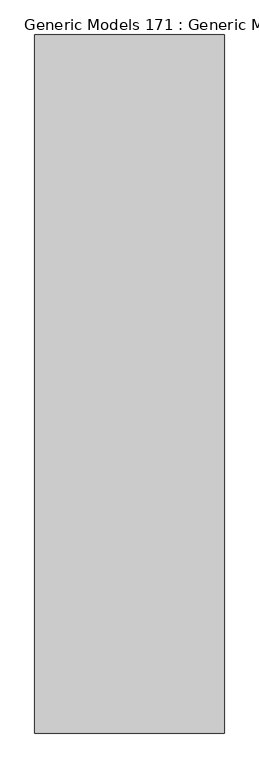
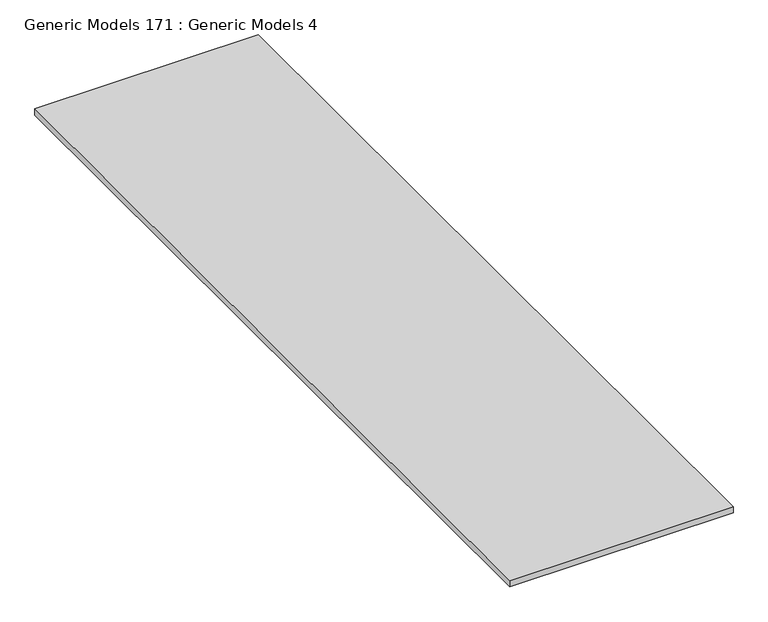
"""IFC4 building model written with IfcOpenShell, lengths in millimetres: proxy geometry, Generic Models 171 : Generic Models 4."""

from ifc_helpers import new_model, si_unit, frame, origin, place, context, project, spatial, polyline, outline, extrude, source, transform, mapped, element, save


def generic_models_171_generic_models_4_48c6cfa5(model_context):
    return source(origin(), model_context, "Body", "SweptSolid", [
        extrude(outline(polyline([(-6629.5736296, -5493.3230338), (-10037.6722239, -5493.3230338), (-10037.6722239, 7054.2769662), (-6629.5736296, 7054.2769662), (-6629.5736296, -5493.3230338)])), frame((0.0, 0.0, 122803.2484874), z_axis=(0.0, 0.0, 1.0), x_axis=(1.0, 0.0, 0.0)), (0.0, 0.0, 1.0), 101.6),
    ])


if __name__ == "__main__":
    model = new_model("IFC4")
    model_context = context("Model", 3, world=origin())
    ifc_project = project(units=[si_unit("LENGTHUNIT", "METRE", prefix="MILLI")], contexts=[model_context])
    site = spatial("IfcSite", under=ifc_project)
    building = spatial("IfcBuilding", under=site)
    placement = place(None, origin())
    generic_models_171_generic_models_4_shape = generic_models_171_generic_models_4_48c6cfa5(model_context)
    element("IfcBuildingElementProxy", 1, Name="Generic Models 171 : Generic Models 4", ObjectType="Generic Models 171 : Generic Models 4", at=placement, inside=building, context=model_context, shape_type="MappedRepresentation", body=[
        mapped(generic_models_171_generic_models_4_shape, transform((0.0, 0.0, 0.0), x_axis=(1.0, 0.0, 0.0), y_axis=(0.0, 1.0, 0.0), z_axis=(0.0, 0.0, 1.0))),
    ])
    save(model, "model.ifc")

# Revit data of these elements
# Element 1 (IfcBuildingElementProxy, "Generic Models 171 : Generic Models 4")
#   Materials on its faces: "_4\" MIN. CRUSHED GRAVEL (NO FINES)"
# Materials
#   "_4\" MIN. CRUSHED GRAVEL (NO FINES)": class "Generic", colour RGB 122 131 148, transparency 0, Cost = 0
